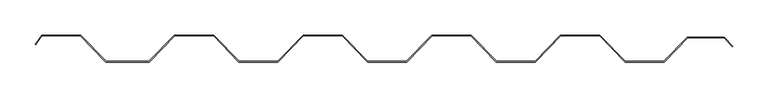
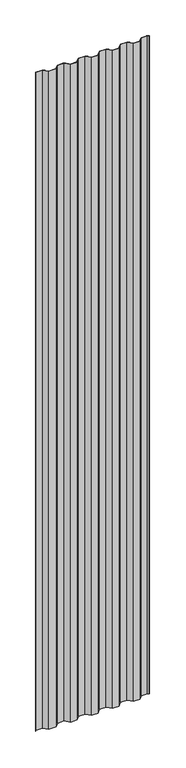
"""IFC4 building model written with IfcOpenShell, lengths in millimetres: proxy geometry, Generic Models 2:Generic Models 2:310765:Generic Models 2:310765 : Generic Models 2:Generic Models 2:310765:2 : Generic Models 2:Generic Models 2:310765:Generic Models 2:310765 : Generic Models 2:Generic Models 2:310765:300385."""

from ifc_helpers import new_model, si_unit, frame, origin, place, context, project, spatial, polyline, outline, extrude, source, transform, mapped, element, save


def generic_models_835397c8(model_context):
    return source(origin(), model_context, "Body", "SweptSolid", [
        extrude(outline(polyline([(593719.8809779, -536496.5394986), (593731.7367242, -536509.6475696), (593731.1747524, -536510.2095414), (593719.5286406, -536497.3332486), (593667.6222866, -536497.3332486), (593633.9903018, -536531.8913358), (593578.8107419, -536531.8913358), (593542.6485503, -536494.5850858), (593487.2734246, -536494.5850858), (593451.111233, -536531.8913358), (593395.9307419, -536531.8913358), (593359.7685503, -536494.5850858), (593304.3934246, -536494.5850858), (593268.231233, -536531.8913358), (593213.0507419, -536531.8913358), (593176.8885503, -536494.5850858), (593121.5134246, -536494.5850858), (593085.351233, -536531.8913358), (593030.1707419, -536531.8913358), (592994.0085503, -536494.5850858), (592938.6334246, -536494.5850858), (592902.471233, -536531.8913358), (592840.9407419, -536531.8913358), (592804.7785503, -536494.5850858), (592750.2499875, -536494.5850858), (592741.3086193, -536507.3546831), (592740.6584173, -536506.8994068), (592749.8367875, -536493.7913358), (592805.1145958, -536493.7913358), (592841.2767875, -536531.0975858), (592902.1351875, -536531.0975858), (592938.2973791, -536493.7913358), (592994.3445958, -536493.7913358), (593030.5067875, -536531.0975858), (593085.0151875, -536531.0975858), (593121.1773791, -536493.7913358), (593177.2245958, -536493.7913358), (593213.3867875, -536531.0975858), (593267.8951875, -536531.0975858), (593304.0573791, -536493.7913358), (593360.1045958, -536493.7913358), (593396.2667875, -536531.0975858), (593450.7751875, -536531.0975858), (593486.9373791, -536493.7913358), (593542.9845958, -536493.7913358), (593579.1467875, -536531.0975858), (593633.6551875, -536531.0975858), (593667.2871722, -536496.5394986), (593719.8809779, -536496.5394986)])), frame((0.0, 0.0, 2463.8), z_axis=(0.0, 0.0, 1.0), x_axis=(1.0, 0.0, 0.0)), (0.0, 0.0, 1.0), 6053.947603),
    ])


if __name__ == "__main__":
    model = new_model("IFC4")
    model_context = context("Model", 3, world=origin())
    ifc_project = project(units=[si_unit("LENGTHUNIT", "METRE", prefix="MILLI")], contexts=[model_context])
    site = spatial("IfcSite", under=ifc_project)
    building = spatial("IfcBuilding", under=site)
    placement = place(None, origin())
    generic_models_shape = generic_models_835397c8(model_context)
    element("IfcBuildingElementProxy", 1, Name="Generic Models 2:Generic Models 2:310765:Generic Models 2:310765 : Generic Models 2:Generic Models 2:310765:2 : Generic Models 2:Generic Models 2:310765:Generic Models 2:310765 : Generic Models 2:Generic Models 2:310765:300385", ObjectType="Generic Models 2:Generic Models 2:310765:Generic Models 2:310765 : Generic Models 2:Generic Models 2:310765:2 : Generic Models 2:Generic Models 2:310765:Generic Models 2:310765 : Generic Models 2:Generic Models 2:310765:300385", at=placement, inside=building, context=model_context, shape_type="MappedRepresentation", body=[
        mapped(generic_models_shape, transform((0.0, 0.0, 0.0), x_axis=(1.0, 0.0, 0.0), y_axis=(0.0, 1.0, 0.0), z_axis=(0.0, 0.0, 1.0))),
    ])
    save(model, "model.ifc")

# Revit data of these elements
# Type "Generic Models 2:Generic Models 2:310765:Generic Models 2:310765 : Generic Models 2:Generic Models 2:310765:2 : Generic Models 2:Generic Models 2:310765:Generic Models 2:310765 : Generic Models 2:Generic Models 2:310765:300385"
#   NameOverride = "Generic Models 2:Generic Models 2:310765:Generic Models 2:310765 : Generic Models 2:Generic Models 2:310765:300385"
#   ObjectTypeOverride = "Generic Models 2:310765 : Generic Models 2:Generic Models 2:310765"
#   Reference = "Generic Models 2"
#   Tag = "300385"
# Element 1 (IfcBuildingElementProxy, "Generic Models 2:Generic Models 2:310765:Generic Models 2:310765 : Generic Models 2:Generic Models 2:310765:2 : Generic Models 2:Generic Models 2:310765:Generic Models 2:310765 : Generic Models 2:Generic Models 2:310765:300385")
#   Materials on its faces: "VERTICAL CORRUGATED METAL PANEL - EXPOSED FASTENERS - (MBCI 7.2 PANEL)"
# Materials
#   "VERTICAL CORRUGATED METAL PANEL - EXPOSED FASTENERS - (MBCI 7.2 PANEL)": class "Generic", colour RGB 120 120 120, transparency 0, Cost = 0
